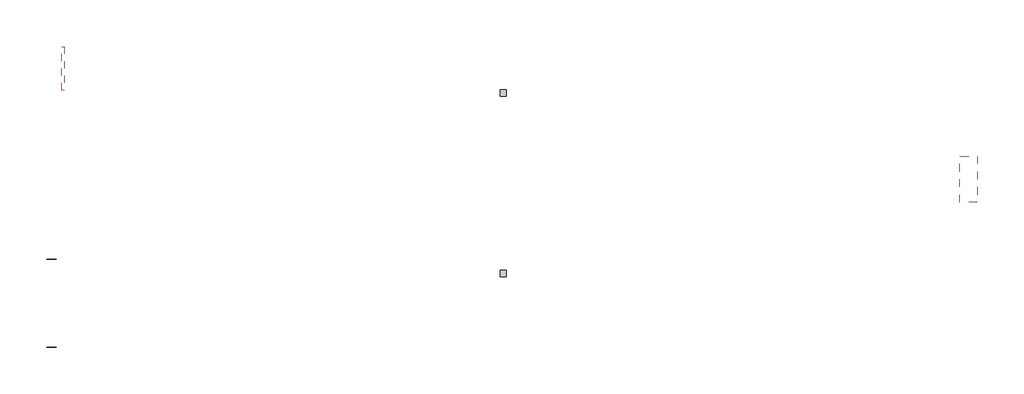
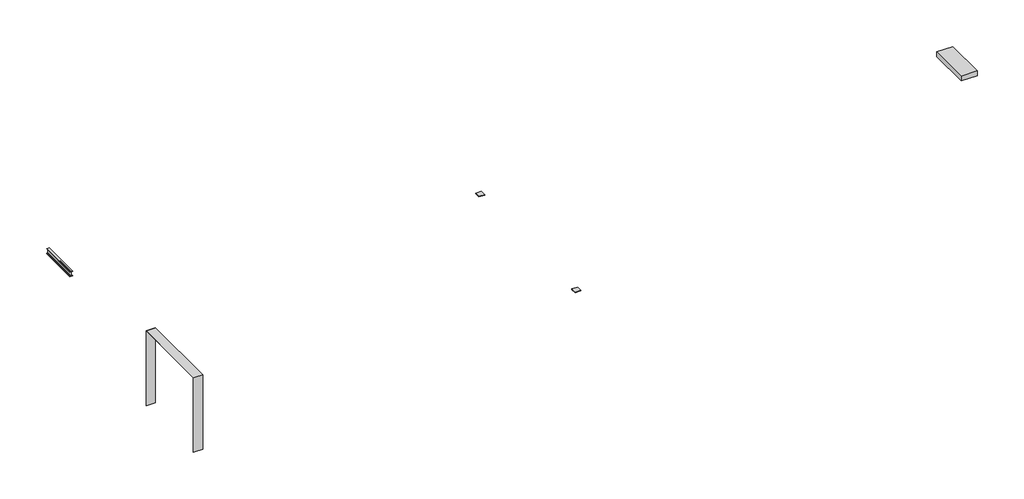
# One storey: 4 proxies, 1 beam.
"""IFC4 building model written with IfcOpenShell, lengths in millimetres."""

import ifcopenshell
import ifcopenshell.guid

model = None  # the IFC model being written
_history = None  # IfcOwnerHistory: only IFC2X3 demands one
_inside = {}  # id of a spatial element -> (the spatial element, [elements in it])
_under = {}  # id of a project, library or spatial element -> (it, [spatial elements below it])
_declared = {}  # id of a project -> (the project, [libraries it declares])
_typed = {}  # id of a type object -> (the type object, [elements of that type])
_made_of = {}  # id of a material, layer set ... -> (it, [elements and type objects made of it])


def new_model(schema):
    """Start an empty IFC model of exactly this schema.

    Asked for "IFC4X3", IfcOpenShell would pick the latest addendum, in which some entities
    have other attributes; the version numbers below select the first issue.
    IFC2X3 requires an IfcOwnerHistory on every rooted entity: one is made here for all.
    """
    global model, _history
    if schema == "IFC4X3":
        model = ifcopenshell.file(schema_version=(4, 3, 0, 0))
    else:
        model = ifcopenshell.file(schema=schema)
    _inside.clear()
    _under.clear()
    _declared.clear()
    _typed.clear()
    _made_of.clear()
    _history = None
    if model.schema == "IFC2X3":
        org = make("IfcOrganization", Name="unknown")
        user = make(
            "IfcPersonAndOrganization",
            ThePerson=make("IfcPerson", FamilyName="unknown"),
            TheOrganization=org,
        )
        app = make(
            "IfcApplication",
            ApplicationDeveloper=org,
            Version="unknown",
            ApplicationFullName="unknown",
            ApplicationIdentifier="unknown",
        )
        _history = make(
            "IfcOwnerHistory",
            OwningUser=user,
            OwningApplication=app,
            ChangeAction="ADDED",
            CreationDate=0,
        )
    return model


def make(cls, **values):
    """One entity of the class cls with the attributes given. An attribute that is None is left unset."""
    return model.create_entity(
        cls, **{name: value for name, value in values.items() if value is not None}
    )


def rooted(cls, **values):
    """An entity with a GlobalId (a new one), such as an element, a storey or a relation."""
    return make(cls, GlobalId=ifcopenshell.guid.new(), OwnerHistory=_history, **values)


def si_unit(unit_type, name, prefix=None):
    """IfcSIUnit, for example si_unit("LENGTHUNIT", "METRE", prefix="MILLI")."""
    return make("IfcSIUnit", UnitType=unit_type, Prefix=prefix, Name=name)


def assignment(units):
    """IfcUnitAssignment: the units of a project."""
    return None if units is None else make("IfcUnitAssignment", Units=units)


def point(xyz):
    """IfcCartesianPoint."""
    return None if xyz is None else make("IfcCartesianPoint", Coordinates=xyz)


def direction(xyz):
    """IfcDirection."""
    return None if xyz is None else make("IfcDirection", DirectionRatios=xyz)


def frame(location, z_axis=None, x_axis=None):
    """IfcAxis2Placement3D, a coordinate frame: its origin and axes. An axis left out is left unset."""
    return make(
        "IfcAxis2Placement3D",
        Location=point(location),
        Axis=direction(z_axis),
        RefDirection=direction(x_axis),
    )


def frame_2d(location, x_axis=None):
    """IfcAxis2Placement2D, a coordinate frame in the plane: its origin and x axis."""
    return make(
        "IfcAxis2Placement2D", Location=point(location), RefDirection=direction(x_axis)
    )


def origin():
    """The frame at (0, 0, 0) with its axes left unset."""
    return frame((0.0, 0.0, 0.0))


def place(relative_to, where):
    """IfcLocalPlacement: puts the frame where relative to a parent placement (None: the world)."""
    return make(
        "IfcLocalPlacement", PlacementRelTo=relative_to, RelativePlacement=where
    )


def context(
    kind, dimensions, precision=None, world=None, true_north=None, identifier=None
):
    """IfcGeometricRepresentationContext, for example the 3D "Model" context."""
    return make(
        "IfcGeometricRepresentationContext",
        ContextIdentifier=identifier,
        ContextType=kind,
        CoordinateSpaceDimension=dimensions,
        Precision=precision,
        WorldCoordinateSystem=world,
        TrueNorth=true_north,
    )


def project(units=None, contexts=None):
    """IfcProject with its units and contexts."""
    return rooted(
        "IfcProject",
        Name="project",
        RepresentationContexts=contexts,
        UnitsInContext=assignment(units),
    )


def spatial(cls, under=None, at=None, **own):
    """A site, building, storey or space (cls), placed at a placement, below another one or the project."""
    s = rooted(cls, ObjectPlacement=at, **own)
    if under is not None:
        _under.setdefault(under.id(), (under, []))[1].append(s)
    return s


def polyline(points):
    """IfcPolyline through the points."""
    return make("IfcPolyline", Points=[point(p) for p in points])


def circle_curve(where, radius):
    """IfcCircle in the frame where."""
    return make("IfcCircle", Position=where, Radius=radius)


def trimmed(basis, trim1, trim2, sense, master):
    """IfcTrimmedCurve: the piece of a basis curve between two trims."""
    return make(
        "IfcTrimmedCurve",
        BasisCurve=basis,
        Trim1=trim1,
        Trim2=trim2,
        SenseAgreement=sense,
        MasterRepresentation=master,
    )


def segment(curve, same_sense, transition):
    """IfcCompositeCurveSegment."""
    return make(
        "IfcCompositeCurveSegment",
        Transition=transition,
        SameSense=same_sense,
        ParentCurve=curve,
    )


def composite_curve(segments, self_intersect=None):
    """IfcCompositeCurve: segments joined end to end."""
    return make("IfcCompositeCurve", Segments=segments, SelfIntersect=self_intersect)


def outline(outer, holes=None, kind="AREA"):
    """IfcArbitraryClosedProfileDef: a profile drawn as a closed curve; with holes, ...WithVoids."""
    if holes is None:
        return make("IfcArbitraryClosedProfileDef", ProfileType=kind, OuterCurve=outer)
    return make(
        "IfcArbitraryProfileDefWithVoids",
        ProfileType=kind,
        OuterCurve=outer,
        InnerCurves=holes,
    )


def extrude(swept, where, along, depth):
    """IfcExtrudedAreaSolid: the profile swept, set in the frame where, extruded along a direction by depth."""
    return make(
        "IfcExtrudedAreaSolid",
        SweptArea=swept,
        Position=where,
        ExtrudedDirection=direction(along),
        Depth=depth,
    )


def shape(context_of_items, identifier, shape_type, items):
    """IfcShapeRepresentation: the items that make up one representation, for example the "Body"."""
    return make(
        "IfcShapeRepresentation",
        ContextOfItems=context_of_items,
        RepresentationIdentifier=identifier,
        RepresentationType=shape_type,
        Items=items,
    )


def source(mapping_origin, context_of_items, identifier, shape_type, items):
    """IfcRepresentationMap: a shape defined once, which mapped items show again and again."""
    return make(
        "IfcRepresentationMap",
        MappingOrigin=mapping_origin,
        MappedRepresentation=shape(context_of_items, identifier, shape_type, items),
    )


def transform(
    local_origin,
    x_axis=None,
    y_axis=None,
    z_axis=None,
    scale=None,
    scale2=None,
    scale3=None,
    uniform=True,
):
    """IfcCartesianTransformationOperator3D, or its non-uniform kind. x_axis, y_axis, z_axis: its Axis1, 2, 3."""
    if uniform:
        return make(
            "IfcCartesianTransformationOperator3D",
            Axis1=direction(x_axis),
            Axis2=direction(y_axis),
            LocalOrigin=point(local_origin),
            Scale=scale,
            Axis3=direction(z_axis),
        )
    return make(
        "IfcCartesianTransformationOperator3DnonUniform",
        Axis1=direction(x_axis),
        Axis2=direction(y_axis),
        LocalOrigin=point(local_origin),
        Scale=scale,
        Axis3=direction(z_axis),
        Scale2=scale2,
        Scale3=scale3,
    )


def mapped(mapping_source, mapping_target):
    """IfcMappedItem: shows the shape of a source again, moved by a transform."""
    return make(
        "IfcMappedItem", MappingSource=mapping_source, MappingTarget=mapping_target
    )


def made_of(thing, what):
    """Note that an element or type object is made of a material, layer set ...; save() writes the relation."""
    if what is not None:
        _made_of.setdefault(what.id(), (what, []))[1].append(thing)
    return thing


def element(
    cls,
    number,
    at=None,
    inside=None,
    cuts=None,
    type_object=None,
    material=None,
    context=None,
    identifier="Body",
    shape_type=None,
    held_by="IfcProductDefinitionShape",
    body=None,
    shapes=None,
    **own,
):
    """One element of the class cls, such as IfcWall. Its Tag is "e" and its number.

    at: its placement. inside: the storey or other place that contains it. cuts: it is an
    opening in that element (IfcRelVoidsElement). A single representation is given by context,
    identifier, shape_type and body (its items); several are given by shapes. held_by: the class
    of the entity that holds the representations. save() writes the other relations.
    """
    e = rooted(cls, Tag="e%d" % number, ObjectPlacement=at, **own)
    if body is not None:
        shapes = [shape(context, identifier, shape_type, body)]
    if shapes is not None:
        e.Representation = make(held_by, Representations=shapes)
    if inside is not None:
        _inside.setdefault(inside.id(), (inside, []))[1].append(e)
    if cuts is not None:
        rooted(
            "IfcRelVoidsElement", RelatingBuildingElement=cuts, RelatedOpeningElement=e
        )
    if type_object is not None:
        _typed.setdefault(type_object.id(), (type_object, []))[1].append(e)
    return made_of(e, material)


def aggregate(whole, parts):
    """IfcRelAggregates: a whole, such as a stair, and the parts it consists of."""
    return rooted("IfcRelAggregates", RelatingObject=whole, RelatedObjects=parts)


def save(model, path):
    """Write the relations noted so far, then the file.

    IfcRelAggregates (storeys below a building ...), IfcRelContainedInSpatialStructure (elements
    in a storey), IfcRelDefinesByType, IfcRelAssociatesMaterial and IfcRelDeclares: one each for
    every whole, place, type object, material and project.
    """
    for whole, parts in _under.values():
        aggregate(whole, parts)
    for where, things in _inside.values():
        rooted(
            "IfcRelContainedInSpatialStructure",
            RelatedElements=things,
            RelatingStructure=where,
        )
    for kind, things in _typed.values():
        rooted("IfcRelDefinesByType", RelatedObjects=things, RelatingType=kind)
    for what, things in _made_of.values():
        rooted("IfcRelAssociatesMaterial", RelatedObjects=things, RelatingMaterial=what)
    for by, libraries in _declared.values():
        rooted("IfcRelDeclares", RelatingContext=by, RelatedDefinitions=libraries)
    model.write(path)


def beam_33eac880(model_context):
    return source(origin(), model_context, "Body", "SweptSolid", [
        extrude(outline(composite_curve([segment(polyline([(82.5, -141.5), (82.5, -151.7), (-82.5, -151.7), (-82.5, -141.5), (-11.9, -141.5)]), True, "CONTINUOUS"), segment(trimmed(circle_curve(frame_2d((-11.9, -132.6)), 8.9), [point((-11.9, -141.5))], [point((-3.0, -132.6))], True, "CARTESIAN"), True, "CONTINUOUS"), segment(polyline([(-3.0, -132.6), (-3.0, 132.6)]), True, "CONTINUOUS"), segment(trimmed(circle_curve(frame_2d((-11.9, 132.6)), 8.9), [point((-3.0, 132.6))], [point((-11.9, 141.5))], True, "CARTESIAN"), True, "CONTINUOUS"), segment(polyline([(-11.9, 141.5), (-82.5, 141.5), (-82.5, 151.7), (82.5, 151.7), (82.5, 141.5), (11.9, 141.5)]), True, "CONTINUOUS"), segment(trimmed(circle_curve(frame_2d((11.9, 132.6)), 8.9), [point((11.9, 141.5))], [point((3.0, 132.6))], True, "CARTESIAN"), True, "CONTINUOUS"), segment(polyline([(3.0, 132.6), (3.0, -132.6)]), True, "CONTINUOUS"), segment(trimmed(circle_curve(frame_2d((11.9, -132.6)), 8.9), [point((3.0, -132.6))], [point((11.9, -141.5))], True, "CARTESIAN"), True, "CONTINUOUS"), segment(polyline([(11.9, -141.5), (82.5, -141.5)]), True, "CONTINUOUS")], self_intersect=False)), frame((-1137.3, 0.0, 0.0), z_axis=(1.0, 0.0, 0.0), x_axis=(0.0, 1.0, 0.0)), (0.0, 0.0, 1.0), 2474.6),
    ])


def generic_models_22d8b4c3(model_context):
    return source(origin(), model_context, "Body", "SweptSolid", [
        extrude(outline(polyline([(25169.0, 25924.5208589), (25169.0, 25574.5208589), (24819.0, 25574.5208589), (24819.0, 25924.5208589), (25169.0, 25924.5208589)])), frame((0.0, 0.0, 863.9720055), z_axis=(0.0, 0.0, 1.0), x_axis=(1.0, 0.0, 0.0)), (0.0, 0.0, 1.0), 36.0),
    ])


def canopy_canopy_9b852544(model_context):
    return source(origin(), model_context, "Body", "SweptSolid", [
        extrude(outline(polyline([(51934.0, 32404.5208589), (51934.0, 29794.5208589), (50934.0, 29794.5208589), (50934.0, 32404.5208589), (51934.0, 32404.5208589)])), frame((0.0, 0.0, 2904.9720055), z_axis=(0.0, 0.0, 1.0), x_axis=(1.0, 0.0, 0.0)), (0.0, 0.0, 1.0), 300.0),
    ])


def generic_models_1_generic_models_1_6dc33216(model_context):
    return source(origin(), model_context, "Body", "SweptSolid", [
        extrude(outline(polyline([(26552.7208589, 1749.9720055), (26551.7208589, 1749.9720055), (26551.7208589, 6598.9720055), (21553.7208589, 6598.9720055), (21553.7208589, 1749.9720055), (21552.7208589, 1749.9720055), (21552.7208589, 6599.9720055), (26552.7208589, 6599.9720055), (26552.7208589, 1749.9720055)])), frame((-935.0, 0.0, 0.0), z_axis=(1.0, 0.0, 0.0), x_axis=(0.0, 1.0, 0.0)), (0.0, 0.0, 1.0), 560.0),
    ])


model = new_model("IFC4")

# Units and contexts
model_context = context("Model", 3, world=origin())
ifc_project = project(units=[si_unit("LENGTHUNIT", "METRE", prefix="MILLI")], contexts=[model_context])

# Site, building, storey
site = spatial("IfcSite", under=ifc_project)
building = spatial("IfcBuilding", under=site)
storey = spatial("IfcBuildingStorey", under=building, Name="B.O.BASE PL.", Elevation=649.9720055)

# Beam
placement = place(None, origin())
beam_shape = beam_33eac880(model_context)
element("IfcBeam", 1, ObjectType="Old_Steel Beam_H-KSD3502 : H_SB_ASB_H-250×125x6x9", at=placement, inside=storey, context=model_context, shape_type="MappedRepresentation", body=[
    mapped(beam_shape, transform((0.0, 37499.5208589, 4148.2720055), x_axis=(0.0, -1.0, 0.0), y_axis=(1.0, 0.0, 0.0), z_axis=(0.0, 0.0, 1.0))),
])

# Proxies
generic_models_shape = generic_models_22d8b4c3(model_context)
element("IfcBuildingElementProxy", 2, Name="플레이트18 : 플레이트", ObjectType="플레이트18 : 플레이트", at=placement, inside=storey, context=model_context, shape_type="MappedRepresentation", body=[
    mapped(generic_models_shape, transform((0.0, 10250.0, -214.0), x_axis=(1.0, 0.0, 0.0), y_axis=(0.0, 1.0, 0.0), z_axis=(0.0, 0.0, 1.0))),
])
element("IfcBuildingElementProxy", 3, Name="플레이트19 : 플레이트", ObjectType="플레이트19 : 플레이트", at=placement, inside=storey, context=model_context, shape_type="MappedRepresentation", body=[
    mapped(generic_models_shape, transform((0.0, 0.0, -214.0), x_axis=(1.0, 0.0, 0.0), y_axis=(0.0, 1.0, 0.0), z_axis=(0.0, 0.0, 1.0))),
])
canopy_canopy_shape = canopy_canopy_9b852544(model_context)
element("IfcBuildingElementProxy", 4, Name="CANOPY : CANOPY", ObjectType="CANOPY : CANOPY", at=placement, inside=storey, context=model_context, shape_type="MappedRepresentation", body=[
    mapped(canopy_canopy_shape, transform((0.0, 0.0, -214.0), x_axis=(1.0, 0.0, 0.0), y_axis=(0.0, 1.0, 0.0), z_axis=(0.0, 0.0, 1.0))),
])
generic_models_1_generic_models_1_shape = generic_models_1_generic_models_1_6dc33216(model_context)
element("IfcBuildingElementProxy", 5, Name="Generic Models 1 : Generic Models 1", ObjectType="Generic Models 1 : Generic Models 1", at=placement, inside=storey, context=model_context, shape_type="MappedRepresentation", body=[
    mapped(generic_models_1_generic_models_1_shape, transform((0.0, 0.0, 0.0), x_axis=(1.0, 0.0, 0.0), y_axis=(0.0, 1.0, 0.0), z_axis=(0.0, 0.0, 1.0))),
])

save(model, "model.ifc")

# Revit data of these elements
# Type "Old_Steel Beam_H-KSD3502 : H_SB_ASB_H-250×125x6x9"
#   Width = 12.5 cm
#   Web Thickness = 0.6 cm
#   Web Fillet = 1.2 cm
#   Warping Constant = 42539.8 cm⁶
#   Torsional Moment of Inertia = 7.8102 cm⁴
#   Torsional Modulus = 1.0 cm³
#   Section Area = 37.66 cm²
#   Plastic Modulus weak axis = 73.1 cm³
#   Plastic Modulus strong axis = 366.0 cm³
#   Perimeter = 0.97 m²/m
#   Nominal Weight = 29.60 kgf/m
#   Moment of Inertia weak axis = 294.00 cm⁴
#   Moment of Inertia strong axis = 4050.00 cm⁴
#   Height = 25.0 cm
#   Flange Thickness = 0.9 cm
#   Elastic Modulus weak axis = 47.0 cm³
#   Elastic Modulus strong axis = 324.0 cm³
#   Centroid Vertical = 12.5 cm
#   Centroid Horizontal = 6.25 cm
#   Length [instance default] = 1.5240 m
#   Structural Material [instance default] = Steel, 45-345
#   Assembly Code = ""
# Element 1 (IfcBeam, "Old_Steel Beam_H-KSD3502 : H_SB_ASB_H-250×125x6x9")
#   Mark = "RSB1"
#   Structural Material = none
#   Phase Created = New Construction
# Element 2 (IfcBuildingElementProxy, "플레이트18 : 플레이트")
#   Phase Created = New Construction
# Element 3 (IfcBuildingElementProxy, "플레이트19 : 플레이트")
#   Phase Created = New Construction
# Element 4 (IfcBuildingElementProxy, "CANOPY : CANOPY")
#   Phase Created = New Construction
# Element 5 (IfcBuildingElementProxy, "Generic Models 1 : Generic Models 1")
#   Phase Created = New Construction
# Materials
#   "Steel, 45-345": class "Metal", colour RGB 189 187 185, transparency 0, Description = "Steel 345 MPa", Cost = 0
